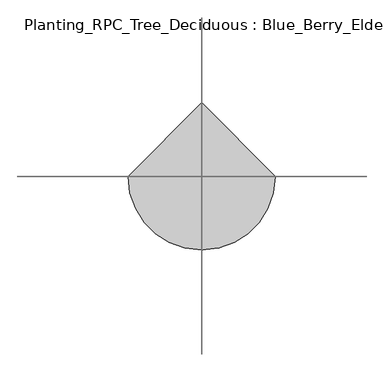
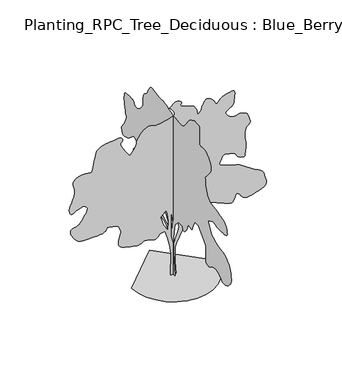
"""IFC4 building model written with IfcOpenShell, lengths in millimetres: geographic element geometry, Planting_RPC_Tree_Deciduous : Blue_Berry_Elder-4.5_Meters."""

from ifc_helpers import new_model, si_unit, origin, place, context, project, spatial, triangles, source, transform, mapped, element, save


def planting_rpc_tree_deciduous_blue_berry_elder_4_5_meters_0b743bd7(model_context):
    return source(origin(), model_context, "Body", "Tessellation", [
        triangles([(-0.0014684, 58.7037978, 0.0041346), (-0.0014684, -62.498052, 0.0041346), (-0.0014684, -15.3641626, 565.6129683), (-0.0014684, -1.8971866, 909.0182064), (-0.0014684, -22.0974929, 1104.2884094), (-0.0014684, -75.9650625, 1326.4911255), (-0.0014684, -224.1009287, 1474.6287403), (-0.0014684, -378.970291, 1474.6287403), (-0.0014684, -412.6378218, 1380.3586224), (-0.0014684, -479.9703761, 1387.0936764), (-0.0014684, -554.0404552, 1474.6287403), (-0.0014684, -601.1729708, 1568.8962421), (-0.0014684, -628.1080273, 1663.1638893), (-0.0014684, -702.1755993, 1636.2313763), (-0.0014684, -782.9756092, 1629.4963223), (-0.0014684, -857.0431812, 1797.8340122), (-0.0014684, -910.9107508, 1898.8340973), (-0.0014684, -1059.0483656, 1892.1015141), (-0.0014684, -1173.5159426, 1797.8340122), (-0.0014684, -1382.2535648, 1575.6288254), (-0.0014684, -1388.9861481, 1353.4261093), (-0.0014684, -1386.9236286, 1327.021035), (-0.0014684, -1382.3910564, 1295.553479), (-0.0014684, -1377.8561588, 1261.3760593), (-0.0014684, -1375.7936394, 1226.8434288), (-0.0014684, -1378.6786377, 1194.3159811), (-0.0014684, -1388.9861481, 1166.1459709), (-0.0014684, -1409.1860779, 1144.6884144), (-0.0014684, -1434.4711624, 1129.1809307), (-0.0014684, -1458.931152, 1117.9109064), (-0.0014684, -1483.3911415, 1111.8258854), (-0.0014684, -1508.676226, 1111.8659266), (-0.0014684, -1535.6112099, 1118.9734142), (-0.0014684, -1565.0162464, 1134.0884073), (-0.0014684, -1597.723843, 1158.1559063), (-0.0014684, -1638.2812511, 1183.6959898), (-0.0014684, -1688.0263252, 1202.5210035), (-0.0014684, -1742.9539318, 1214.5159836), (-0.0014684, -1799.0589375, 1219.5610245), (-0.0014684, -1852.3364994, 1217.541017), (-0.0014684, -1898.7841003, 1208.3335121), (-0.0014684, -1934.3939907, 1191.8234734), (-0.0014684, -1963.8416119, 1167.0484594), (-0.0014684, -1995.1716763, 1136.2684341), (-0.0014684, -2029.446619, 1104.1908863), (-0.0014684, -2067.729166, 1075.5283916), (-0.0014684, -2111.0741947, 1054.9958513), (-0.0014684, -2160.5442856, 1047.2983561), (-0.0014684, -2217.1992577, 1057.1533504), (-0.0014684, -2275.1493542, 1083.4008762), (-0.0014684, -2327.0944393, 1119.5408941), (-0.0014684, -2371.9694618, 1162.2784744), (-0.0014684, -2408.7193989, 1208.3134552), (-0.0014684, -2436.2819607, 1254.3485813), (-0.0014684, -2453.5944214, 1297.0836182), (-0.0014684, -2459.6019035, 1333.2260342), (-0.0014684, -2455.754464, 1372.7236233), (-0.0014684, -2445.3120781, 1424.1161259), (-0.0014684, -2429.919413, 1481.9887562), (-0.0014684, -2411.2318909, 1540.9212055), (-0.0014684, -2390.8944695, 1595.4962173), (-0.0014684, -2370.5569027, 1640.2937737), (-0.0014684, -2351.8669098, 1669.8963272), (-0.0014684, -2330.1568977, 1694.4363991), (-0.0014684, -2300.199424, 1725.2163517), (-0.0014684, -2262.8217636, 1758.5913494), (-0.0014684, -2218.8493023, 1790.903912), (-0.0014684, -2169.1042282, 1818.5039715), (-0.0014684, -2114.4116364, 1837.74146), (-0.0014684, -2055.5966217, 1844.9664551), (-0.0014684, -1994.4066067, 1849.8740044), (-0.0014684, -1932.1566273, 1863.6164795), (-0.0014684, -1869.0239983, 1884.7189705), (-0.0014684, -1805.1839996, 1911.7115089), (-0.0014684, -1740.8139462, 1943.1215103), (-0.0014684, -1676.0888271, 1977.4765354), (-0.0014684, -1611.1888641, 2013.3016743), (-0.0014684, -1469.786158, 2275.9068661), (-0.0014684, -1685.2562908, 2376.9094219), (-0.0014684, -1714.2713802, 2368.3093655), (-0.0014684, -1744.228854, 2360.0643745), (-0.0014684, -1776.0713871, 2352.5268986), (-0.0014684, -1810.7388931, 2346.049387), (-0.0014684, -1849.1765179, 2340.9844345), (-0.0014684, -1892.3265003, 2337.686816), (-0.0014684, -1941.1290447, 2336.5069462), (-0.0014684, -1996.881601, 2336.291843), (-0.0014684, -2057.3441895, 2336.4293346), (-0.0014684, -2118.1616982, 2338.0968201), (-0.0014684, -2174.9742188, 2342.4769306), (-0.0014684, -2223.421843, 2350.7393623), (-0.0014684, -2259.1517841, 2364.0693626), (-0.0014684, -2277.7993378, 2383.6418598), (-0.0014684, -2281.3744102, 2414.4819832), (-0.0014684, -2275.8767807, 2457.2194908), (-0.0014684, -2262.9592552, 2506.4269524), (-0.0014684, -2244.2692623, 2556.7020813), (-0.0014684, -2221.4593174, 2602.6271851), (-0.0014684, -2196.1742329, 2638.7770134), (-0.0014684, -2170.0641987, 2659.7021896), (-0.0014684, -2143.7192951, 2670.2021301), (-0.0014684, -2115.1367374, 2679.2771576), (-0.0014684, -2082.0791622, 2687.9772079), (-0.0014684, -2042.3065899, 2697.4022141), (-0.0014684, -1993.581657, 2708.6021118), (-0.0014684, -1933.6665642, 2722.6021294), (-0.0014684, -1860.326564, 2740.5021996), (-0.0014684, -1781.7239491, 2758.3022758), (-0.0014684, -1708.0688519, 2773.1522415), (-0.0014684, -1640.1838966, 2787.8522163), (-0.0014684, -1578.8962132, 2805.302314), (-0.0014684, -1525.0287163, 2828.2773651), (-0.0014684, -1479.4062103, 2859.6021973), (-0.0014684, -1442.8536449, 2902.1272179), (-0.0014684, -1414.8411106, 2953.5272781), (-0.0014684, -1393.5411026, 3009.1773697), (-0.0014684, -1377.8361019, 3068.3775352), (-0.0014684, -1366.6061188, 3130.3775299), (-0.0014684, -1358.7336342, 3194.527684), (-0.0014684, -1353.1011292, 3260.0777527), (-0.0014684, -1348.5861431, 3326.3277786), (-0.0014684, -1398.7811897, 3378.2528069), (-0.0014684, -1447.1536732, 3430.0528427), (-0.0014684, -1491.8711472, 3481.6278923), (-0.0014684, -1531.1136646, 3532.8529633), (-0.0014684, -1563.0537209, 3583.577774), (-0.0014684, -1585.8662819, 3633.7529091), (-0.0014684, -1597.723843, 3683.2030884), (-0.0014684, -1593.7188549, 3737.8779488), (-0.0014684, -1572.2812099, 3799.8529449), (-0.0014684, -1536.5912373, 3863.2281464), (-0.0014684, -1489.8311554, 3922.153038), (-0.0014684, -1435.1786774, 3970.7032722), (-0.0014684, -1375.8135509, 4002.9783371), (-0.0014684, -1314.918576, 4013.128299), (-0.0014684, -1258.4585049, 4010.1031929), (-0.0014684, -1210.3634754, 4007.7533363), (-0.0014684, -1170.7484516, 4007.6533424), (-0.0014684, -1139.7309408, 4011.3281181), (-0.0014684, -1117.4309212, 4020.3031517), (-0.0014684, -1103.9633566, 4036.1033501), (-0.0014684, -1099.4483706, 4060.2783279), (-0.0014684, -1101.1558971, 4105.3531929), (-0.0014684, -1104.8659178, 4175.1532928), (-0.0014684, -1108.4584311, 4258.1534592), (-0.0014684, -1109.8133629, 4342.8035248), (-0.0014684, -1106.8083864, 4417.5536133), (-0.0014684, -1097.3283691, 4470.8785561), (-0.0014684, -1079.2483681, 4491.2037689), (-0.0014684, -1052.7858845, 4492.578685), (-0.0014684, -1020.9033102, 4495.6035004), (-0.0014684, -985.6082989, 4498.6286064), (-0.0014684, -948.8982576, 4500.0035225), (-0.0014684, -912.7757532, 4498.07864), (-0.0014684, -879.2456778, 4491.2037689), (-0.0014684, -850.3106707, 4477.7537178), (-0.0014684, -822.8281912, 4461.7535316), (-0.0014684, -792.8706448, 4447.2035477), (-0.0014684, -761.2631264, 4432.1535942), (-0.0014684, -728.8330564, 4414.7534935), (-0.0014684, -696.4030592, 4393.1286507), (-0.0014684, -664.7980116, 4365.3786003), (-0.0014684, -634.8405378, 4329.6034584), (-0.0014684, -604.8054889, 4286.4284775), (-0.0014684, -572.6504748, 4239.8534134), (-0.0014684, -538.7279451, 4193.0283646), (-0.0014684, -503.3904219, 4149.1534264), (-0.0014684, -466.9953687, 4111.403405), (-0.0014684, -429.8928369, 4082.9533974), (-0.0014684, -392.4378193, 4067.0032082), (-0.0014684, -354.0977903, 4061.0282822), (-0.0014684, -314.1102602, 4059.6533661), (-0.0014684, -272.4727218, 4061.703241), (-0.0014684, -229.1851932, 4065.9782707), (-0.0014684, -184.2498909, 4071.3282349), (-0.0014684, -137.6653616, 4076.5532066), (-0.0014684, -89.4320684, 4080.4782578), (-0.0014684, -32.5020268, 4087.803392), (-0.0014684, 35.3820291, 4102.1033913), (-0.0014684, 107.0353362, 4120.403437), (-0.0014684, 175.2726409, 4139.7534187), (-0.0014684, 232.909439, 4157.2282242), (-0.0014684, 272.7602224, 4169.8783241), (-0.0014684, 287.6402371, 4174.7283188), (-0.0014684, 295.8277461, 4177.2784538), (-0.0014684, 318.5002539, 4183.6033585), (-0.0014684, 352.8352947, 4191.7034454), (-0.0014684, 396.002827, 4199.553257), (-0.0014684, 445.1803485, 4205.1534966), (-0.0014684, 497.5354013, 4206.5284126), (-0.0014684, 550.2454471, 4201.678418), (-0.0014684, 608.3329988, 4200.728476), (-0.0014684, 675.2555128, 4211.4534027), (-0.0014684, 745.8280947, 4228.1785446), (-0.0014684, 814.8706827, 4245.2533745), (-0.0014684, 877.2007444, 4257.0285278), (-0.0014684, 927.6307331, 4257.8534775), (-0.0014684, 960.9857466, 4242.0785683), (-0.0014684, 983.9932812, 4214.9534798), (-0.0014684, 1006.5283155, 4185.8035149), (-0.0014684, 1028.1233637, 4155.1533508), (-0.0014684, 1048.3033819, 4123.4282524), (-0.0014684, 1066.5983408, 4091.1031906), (-0.0014684, 1082.5408997, 4058.6781349), (-0.0014684, 1095.6533987, 4026.6033485), (-0.0014684, 1111.3184309, 3999.2282753), (-0.0014684, 1133.5808802, 3978.353096), (-0.0014684, 1159.9634268, 3960.5283119), (-0.0014684, 1187.9984888, 3942.3532585), (-0.0014684, 1215.2059851, 3920.4031448), (-0.0014684, 1239.1159355, 3891.2531799), (-0.0014684, 1257.255962, 3851.5279884), (-0.0014684, 1268.2685165, 3817.1530518), (-0.0014684, 1273.6285091, 3800.8031776), (-0.0014684, 1275.1010937, 3794.1030052), (-0.0014684, 1274.4534588, 3788.7030441), (-0.0014684, 1273.451049, 3776.252932), (-0.0014684, 1273.8635239, 3748.3528908), (-0.0014684, 1277.4560371, 3696.6528488), (-0.0014684, 1283.7985279, 3637.6029648), (-0.0014684, 1291.9060272, 3591.1778915), (-0.0014684, 1302.7210648, 3554.2528198), (-0.0014684, 1317.1884956, 3523.8279327), (-0.0014684, 1336.2511402, 3496.8278366), (-0.0014684, 1360.8486214, 3470.1527206), (-0.0014684, 1391.9260849, 3440.8027679), (-0.0014684, 1427.2211689, 3411.5778076), (-0.0014684, 1463.2262386, 3387.677813), (-0.0014684, 1498.9912067, 3369.4027657), (-0.0014684, 1533.5812466, 3357.1526413), (-0.0014684, 1566.0512123, 3351.2777092), (-0.0014684, 1595.4587196, 3352.1026588), (-0.0014684, 1620.8612389, 3360.002758), (-0.0014684, 1639.7087803, 3375.502684), (-0.0014684, 1652.8988182, 3396.6528465), (-0.0014684, 1664.6789131, 3420.0528717), (-0.0014684, 1679.2838356, 3442.2776779), (-0.0014684, 1700.9563499, 3459.9027649), (-0.0014684, 1733.936459, 3469.5277588), (-0.0014684, 1782.4638748, 3467.7278687), (-0.0014684, 1840.5514629, 3464.2277916), (-0.0014684, 1897.5815575, 3466.9779144), (-0.0014684, 1950.8390625, 3469.852739), (-0.0014684, 1997.6216721, 3466.7029312), (-0.0014684, 2035.2141449, 3451.4277008), (-0.0014684, 2060.9117043, 3417.9027122), (-0.0014684, 2072.001725, 3360.002758), (-0.0014684, 2074.396637, 3302.2527946), (-0.0014684, 2075.4967152, 3266.6526421), (-0.0014684, 2074.8291687, 3243.2026199), (-0.0014684, 2071.9241135, 3221.8774681), (-0.0014684, 2066.3091946, 3192.6275093), (-0.0014684, 2057.5140919, 3145.5024788), (-0.0014684, 2045.069212, 3070.4524086), (-0.0014684, 2028.7941879, 2993.7774376), (-0.0014684, 2011.3440903, 2941.8274109), (-0.0014684, 1996.4816254, 2904.7273499), (-0.0014684, 1987.9815628, 2872.5772774), (-0.0014684, 1989.6115505, 2835.4772163), (-0.0014684, 2005.1390911, 2783.5271896), (-0.0014684, 2038.3341579, 2706.8522186), (-0.0014684, 2081.1517479, 2626.4521843), (-0.0014684, 2121.139278, 2566.6770538), (-0.0014684, 2155.4742462, 2522.5771294), (-0.0014684, 2181.326738, 2489.1794586), (-0.0014684, 2195.8742512, 2461.5570168), (-0.0014684, 2196.286726, 2434.7619953), (-0.0014684, 2179.7367187, 2403.841935), (-0.0014684, 2160.4392048, 2371.8244125), (-0.0014684, 2149.859182, 2345.5768867), (-0.0014684, 2141.0441677, 2325.9269234), (-0.0014684, 2127.0467663, 2313.6968559), (-0.0014684, 2100.919146, 2309.7119247), (-0.0014684, 2055.7091148, 2314.7969341), (-0.0014684, 1984.4666611, 2329.7743629), (-0.0014684, 1906.7291096, 2358.6118469), (-0.0014684, 1844.06651, 2399.6994553), (-0.0014684, 1792.5939251, 2445.4995667), (-0.0014684, 1748.4239468, 2488.4719437), (-0.0014684, 1707.671347, 2521.0769302), (-0.0014684, 1666.4437763, 2535.7769051), (-0.0014684, 1620.8612389, 2525.0519783), (-0.0014684, 1576.9088345, 2499.6619583), (-0.0014684, 1542.1411892, 2475.3396057), (-0.0014684, 1515.031216, 2451.8994667), (-0.0014684, 1494.0461597, 2429.166988), (-0.0014684, 1477.653701, 2406.9644188), (-0.0014684, 1464.3237007, 2385.1144444), (-0.0014684, 1452.526165, 2363.44193), (-0.0014684, 1471.2737125, 2344.7718487), (-0.0014684, 1489.9612347, 2326.6344383), (-0.0014684, 1508.5336475, 2309.5543762), (-0.0014684, 1526.9262749, 2294.0668041), (-0.0014684, 1545.0862129, 2280.6968353), (-0.0014684, 1562.9512562, 2269.9793209), (-0.0014684, 1580.4612339, 2262.4393742), (-0.0014684, 1599.1313152, 2259.024321), (-0.0014684, 1619.331245, 2258.1993713), (-0.0014684, 1639.2963055, 2256.7868122), (-0.0014684, 1657.2588718, 2251.6042797), (-0.0014684, 1671.4513195, 2239.4718807), (-0.0014684, 1680.1087852, 2217.2092861), (-0.0014684, 1681.4637897, 2181.6392189), (-0.0014684, 1676.9863014, 2141.9842266), (-0.0014684, 1669.5664055, 2107.6292015), (-0.0014684, 1659.5537899, 2075.631736), (-0.0014684, 1647.3038109, 2043.0441902), (-0.0014684, 1633.1713886, 2006.9216858), (-0.0014684, 1617.5037403, 1964.3241405), (-0.0014684, 1600.6613091, 1912.3015892), (-0.0014684, 1583.268766, 1853.7415009), (-0.0014684, 1567.0537674, 1795.0639778), (-0.0014684, 1554.0188072, 1738.6264343), (-0.0014684, 1546.1662342, 1686.7788723), (-0.0014684, 1545.4986877, 1641.8837929), (-0.0014684, 1554.0188072, 1606.2938141), (-0.0014684, 1573.728796, 1582.3637341), (-0.0014684, 1599.1112583, 1566.4212479), (-0.0014684, 1623.4337563, 1552.9562267), (-0.0014684, 1646.8738953, 1541.5487835), (-0.0014684, 1669.606374, 1531.7937103), (-0.0014684, 1691.8087978, 1523.2737362), (-0.0014684, 1713.6589176, 1515.5787117), (-0.0014684, 1735.331432, 1508.2936913), (-0.0014684, 1758.2389, 1518.0512352), (-0.0014684, 1780.0888744, 1525.7462597), (-0.0014684, 1799.8189201, 1529.318716), (-0.0014684, 1816.3664566, 1526.7087009), (-0.0014684, 1828.676461, 1515.8536949), (-0.0014684, 1835.6840275, 1494.6911785), (-0.0014684, 1836.331517, 1461.1612484), (-0.0014684, 1830.501495, 1425.4711304), (-0.0014684, 1819.3715057, 1398.2636341), (-0.0014684, 1803.8239082, 1378.1211136), (-0.0014684, 1784.7414974, 1363.6336258), (-0.0014684, 1763.0089577, 1353.3861408), (-0.0014684, 1739.5114094, 1345.9660995), (-0.0014684, 1715.128886, 1339.9586174), (-0.0014684, 1703.5663651, 1332.6360992), (-0.0014684, 1691.8864094, 1324.6660915), (-0.0014684, 1679.9712936, 1315.4011047), (-0.0014684, 1667.701403, 1304.1910332), (-0.0014684, 1654.9613377, 1290.3910034), (-0.0014684, 1641.6313374, 1273.3510551), (-0.0014684, 1627.5962929, 1252.4235535), (-0.0014684, 1608.2588104, 1230.1234612), (-0.0014684, 1580.0887276, 1209.2360006), (-0.0014684, 1544.5563034, 1189.5259392), (-0.0014684, 1503.1336864, 1170.7584801), (-0.0014684, 1457.2962227, 1152.6984632), (-0.0014684, 1408.5135899, 1135.1084032), (-0.0014684, 1358.2586632, 1117.7559013), (-0.0014684, 1196.6559546, 1212.0234758), (-0.0014684, 1035.0533186, 1090.8208448), (-0.0014684, 1013.4382862, 1088.0133854), (-0.0014684, 992.0007866, 1085.6783535), (-0.0014684, 970.9182798, 1084.2833805), (-0.0014684, 950.3632845, 1084.3033648), (-0.0014684, 930.5182749, 1086.2084084), (-0.0014684, 911.5532261, 1090.4683954), (-0.0014684, 893.6507578, 1097.5558989), (-0.0014684, 877.0431959, 1106.938393), (-0.0014684, 861.3756929, 1117.3809242), (-0.0014684, 845.9456755, 1128.295883), (-0.0014684, 830.0457012, 1139.0934071), (-0.0014684, 812.9656391, 1149.1834162), (-0.0014684, 794.0031338, 1157.9784462), (-0.0014684, 772.4481268, 1164.8884169), (-0.0014684, 748.1855816, 1170.2684664), (-0.0014684, 721.8005642, 1174.9409283), (-0.0014684, 693.6505383, 1179.0234552), (-0.0014684, 664.0855551, 1182.6359528), (-0.0014684, 633.4605349, 1185.8934574), (-0.0014684, 602.1304705, 1188.9184908), (-0.0014684, 570.4454495, 1191.8234734), (-0.0014684, 361.7077909, 1131.2209225), (-0.0014684, 186.6391528, 1003.2857809), (-0.0014684, 92.3710787, 848.418199), (-0.0014684, 45.2367873, 552.1454401), (-0.0013758, 65.4370532, 1097.5558989), (-0.0013758, 166.4388778, 1313.0261044), (-0.0013758, 4.8361539, 1380.3586224), (-0.0013882, 307.8402577, 1171.6234709), (-0.0013882, 469.4428937, 1279.3585373), (-0.0013882, 597.3779989, 1286.0909752), (-0.0013882, 705.1130653, 1346.6910553), (-0.0013882, 699.3031002, 1349.8135391), (-0.0013882, 693.2555769, 1354.3485821), (-0.0013882, 686.7405676, 1361.7110687), (-0.0013882, 679.5155725, 1373.3110874), (-0.0013882, 671.3480478, 1390.5686096), (-0.0013882, 662.0055222, 1414.8911076), (-0.0013882, 651.2454958, 1447.6936111), (-0.0013882, 642.6479828, 1480.1036968), (-0.0013882, 639.3505096, 1503.3287327), (-0.0013882, 640.4680286, 1518.8962418), (-0.0013882, 645.1205063, 1528.3386887), (-0.0013882, 652.425511, 1533.1862125), (-0.0013882, 661.4930534, 1534.9737488), (-0.0013882, 671.4480417, 1535.2286751), (-0.0013882, 678.1805523, 1616.0288303), (-0.0013882, 597.3779989, 1669.8963272), (-0.0013882, 422.3103418, 1521.7611832), (-0.0013882, 301.1077472, 1380.3586224), (-0.0013882, 220.3061749, 1265.8910454), (-0.0013882, 139.504866, 1084.0884069), (66.6360534, 0.0002629, 0.0), (-68.0330566, 0.0002629, 0.0), (-61.2998012, 0.0002272, 552.142933), (-94.9670776, 0.0002139, 794.5456152), (-142.1008648, 0.0002005, 996.5483288), (-202.7016716, 0.0001916, 1178.3509672), (-323.9027584, 0.0001916, 1164.8859461), (-344.1627863, 0.0001916, 1136.3209019), (-364.7752999, 0.000196, 1109.5258804), (-386.0953285, 0.000196, 1086.2633469), (-408.4753215, 0.000196, 1068.3008532), (-432.2678372, 0.0002005, 1057.4058786), (-457.8253615, 0.0002005, 1055.3433592), (-485.5053944, 0.000196, 1063.8833902), (-514.9529065, 0.000196, 1076.7408903), (-545.4604557, 0.000196, 1086.7733448), (-576.8504728, 0.000196, 1094.448385), (-608.9454978, 0.000196, 1100.2409094), (-641.5730484, 0.000196, 1104.6184038), (-674.5530121, 0.000196, 1108.0533686), (-707.7105812, 0.000196, 1111.0183765), (-735.2131176, 0.000196, 1095.3133759), (-763.2456362, 0.000196, 1080.6083868), (-792.3406626, 0.000196, 1067.9083626), (-823.0231647, 0.000196, 1058.210844), (-855.8256683, 0.0002005, 1052.5183863), (-891.280699, 0.0002005, 1051.8308556), (-929.9132246, 0.0002005, 1057.1508797), (-979.8558157, 0.000196, 1066.7883728), (-1044.1658438, 0.000196, 1079.0183676), (-1115.7808765, 0.000196, 1094.7833937), (-1187.630924, 0.000196, 1115.0233646), (-1252.6485397, 0.0001916, 1140.6809555), (-1303.7660591, 0.0001916, 1172.6984779), (-1333.9185791, 0.0001871, 1212.0184616), (-1343.6560661, 0.0001871, 1258.8785374), (-1340.9085594, 0.0001827, 1310.6835148), (-1329.6785763, 0.0001782, 1364.141153), (-1313.9735756, 0.0001782, 1415.9461304), (-1297.7985455, 0.0001738, 1462.8062061), (-1285.1560032, 0.0001738, 1501.4186749), (-1280.0510822, 0.0001693, 1528.4912956), (-1282.3885849, 0.0001693, 1551.6362492), (-1288.8460396, 0.0001693, 1579.2562202), (-1298.6035835, 0.0001648, 1609.2337509), (-1310.8335056, 0.0001648, 1639.4462963), (-1324.7136177, 0.0001604, 1667.7737823), (-1339.4160633, 0.0001604, 1692.0964256), (-1354.121125, 0.0001604, 1710.2938614), (-1373.4561367, 0.0001604, 1723.3488785), (-1401.6286903, 0.0001559, 1733.9289013), (-1437.1586437, 0.0001559, 1742.4488754), (-1478.5812607, 0.0001559, 1749.3189503), (-1524.4187244, 0.0001559, 1754.9539261), (-1573.2012119, 0.0001559, 1759.7639523), (-1623.456284, 0.0001559, 1764.1613583), (-1631.2713593, 0.0001559, 1738.3664211), (-1642.6763317, 0.0001604, 1713.6314484), (-1661.2663307, 0.0001604, 1691.0164043), (-1690.6363403, 0.0001604, 1671.5813988), (-1734.3739323, 0.0001604, 1656.386396), (-1796.0739452, 0.0001648, 1646.4938313), (-1879.3290379, 0.0001648, 1642.9588726), (-1971.5741341, 0.0001648, 1640.6613384), (-2057.4616241, 0.0001648, 1636.1262955), (-2136.396777, 0.0001648, 1632.8888477), (-2207.7943085, 0.0001648, 1634.478867), (-2271.0668999, 0.0001648, 1644.4313118), (-2325.619384, 0.0001604, 1666.2812862), (-2370.8693836, 0.0001604, 1703.5614235), (-2411.8019142, 0.0001559, 1752.5588688), (-2450.9643494, 0.0001559, 1805.3264328), (-2484.1219185, 0.0001515, 1859.0389973), (-2507.0269157, 0.000147, 1910.8640316), (-2515.4519829, 0.0001426, 1957.9790337), (-2505.1520302, 0.0001426, 1997.554089), (-2471.8720848, 0.0001426, 2026.7640793), (-2428.4670307, 0.0001381, 2045.1192089), (-2390.1269291, 0.0001381, 2056.5266521), (-2356.1468811, 0.0001381, 2064.7517315), (-2325.816901, 0.0001381, 2073.5667458), (-2298.4317993, 0.0001381, 2086.7391975), (-2273.2843517, 0.0001337, 2108.0367348), (-2249.6667526, 0.0001337, 2141.2342724), (-2221.7142437, 0.0001292, 2184.9518074), (-2187.6342018, 0.0001292, 2233.7342949), (-2152.8467903, 0.0001247, 2285.2267914), (-2122.7717365, 0.0001203, 2337.0718826), (-2102.826733, 0.0001203, 2386.9169506), (-2098.4291817, 0.0001158, 2432.401965), (-2114.9992458, 0.0001158, 2471.1721275), (-2145.426749, 0.0001114, 2498.537027), (-2178.6816959, 0.0001114, 2512.8271431), (-2214.2917316, 0.0001114, 2516.2269356), (-2251.7868267, 0.0001114, 2510.9019699), (-2290.6968063, 0.0001114, 2499.0494957), (-2330.5468449, 0.0001114, 2482.831881), (-2370.8693836, 0.0001158, 2464.439399), (-2399.569376, 0.0001158, 2448.8118645), (-2427.3294548, 0.0001158, 2434.6595306), (-2453.2020035, 0.0001158, 2423.4494591), (-2476.2471085, 0.0001158, 2416.6569958), (-2495.5270363, 0.0001158, 2415.7544346), (-2510.1020187, 0.0001158, 2422.2118893), (-2519.0020569, 0.0001158, 2437.5044151), (-2525.7269371, 0.0001158, 2456.4494797), (-2533.1520653, 0.0001158, 2474.4518692), (-2539.5019684, 0.0001114, 2493.8669632), (-2543.0270439, 0.0001114, 2517.0521759), (-2541.977108, 0.0001114, 2546.3521317), (-2534.5519798, 0.0001069, 2584.15215), (-2519.0020569, 0.0001025, 2632.7770889), (-2498.1969315, 0.0001025, 2684.6521202), (-2477.0345604, 9.8e-05, 2732.0771324), (-2456.8145737, 9.8e-05, 2777.1272896), (-2438.8319504, 9.36e-05, 2821.9271713), (-2424.3844311, 8.91e-05, 2868.6522263), (-2414.7643787, 8.91e-05, 2919.3523293), (-2411.2693886, 8.47e-05, 2976.1773491), (-2415.2169674, 8.02e-05, 3030.6775108), (-2424.696912, 8.02e-05, 3074.9274261), (-2436.1819668, 7.57e-05, 3111.8774963), (-2446.1344116, 7.57e-05, 3144.4525429), (-2451.0245201, 7.13e-05, 3175.6276749), (-2447.311956, 7.13e-05, 3208.3277138), (-2431.4719345, 6.68e-05, 3245.527478), (-2401.6519524, 6.68e-05, 3281.1526291), (-2361.1144558, 6.24e-05, 3307.9527374), (-2313.9793968, 6.24e-05, 3326.977739), (-2264.3718143, 6.24e-05, 3339.2775696), (-2216.4142765, 6.24e-05, 3345.9277451), (-2174.2267353, 6.24e-05, 3348.0026184), (-2141.9342297, 6.24e-05, 3346.5277084), (-2114.2341763, 6.24e-05, 3341.002755), (-2084.4141941, 6.24e-05, 3332.902668), (-2054.4766319, 6.24e-05, 3326.2027863), (-2026.4241291, 6.24e-05, 3324.9275734), (-2002.2565636, 6.24e-05, 3333.0776573), (-1983.9816616, 6.24e-05, 3354.6527939), (-1973.5965397, 5.79e-05, 3393.652739), (-1964.8216393, 5.35e-05, 3450.0277863), (-1951.2165104, 5.35e-05, 3517.3777451), (-1934.5515392, 4.9e-05, 3590.1279556), (-1916.5891182, 4.46e-05, 3662.7528831), (-1899.0965813, 4.01e-05, 3729.7281555), (-1883.8440239, 3.56e-05, 3785.5279472), (-1872.5939838, 3.12e-05, 3824.6031784), (-1852.5114887, 3.12e-05, 3852.8781967), (-1813.3489082, 3.12e-05, 3879.4030312), (-1760.7564789, 2.67e-05, 3903.2280304), (-1700.3914135, 2.67e-05, 3923.3782539), (-1637.906274, 2.67e-05, 3938.9531754), (-1578.9537678, 2.67e-05, 3948.9781448), (-1529.1887821, 2.67e-05, 3952.5282188), (-1482.7811497, 2.67e-05, 3955.978299), (-1432.4861092, 2.67e-05, 3963.6781197), (-1381.8386192, 2.67e-05, 3971.6032173), (-1334.3710224, 2.23e-05, 3975.7782532), (-1293.6160973, 2.67e-05, 3972.1531837), (-1263.1109825, 2.67e-05, 3956.7782501), (-1246.3835152, 2.67e-05, 3925.6031181), (-1245.9735111, 3.12e-05, 3891.2531799), (-1257.1035004, 3.12e-05, 3865.2780212), (-1272.3560577, 3.12e-05, 3842.0279869), (-1284.3134674, 3.56e-05, 3815.8281326), (-1285.5485664, 3.56e-05, 3781.0029327), (-1268.6459644, 4.01e-05, 3731.9530197), (-1226.1860561, 4.46e-05, 3663.0028679), (-1175.7534513, 4.9e-05, 3589.303006), (-1137.6884056, 4.9e-05, 3530.2028343), (-1108.6933731, 5.35e-05, 3486.3028976), (-1085.4708807, 5.35e-05, 3458.2028687), (-1064.7208391, 5.79e-05, 3446.4527138), (-1043.1458479, 5.35e-05, 3451.6776855), (-1017.4482885, 5.35e-05, 3474.4527489), (-990.2407923, 5.35e-05, 3507.3527756), (-966.3282984, 4.9e-05, 3542.2529709), (-945.7157484, 4.9e-05, 3578.7027809), (-928.403215, 4.46e-05, 3616.2028175), (-914.3857567, 4.46e-05, 3654.2778191), (-903.6682423, 4.01e-05, 3692.4781036), (-896.2457302, 4.01e-05, 3730.3281189), (-882.6607309, 3.56e-05, 3773.9530724), (-855.1781788, 3.12e-05, 3826.1530838), (-816.3881773, 3.12e-05, 3881.5531906), (-768.880612, 2.67e-05, 3934.7281425), (-715.2480572, 2.23e-05, 3980.2282722), (-658.0830145, 2.23e-05, 4012.6533279), (-599.9754785, 2.23e-05, 4026.6033485), (-552.8204352, 2.23e-05, 4024.7781693), (-521.215424, 2.23e-05, 4016.1031174), (-496.7928958, 2.23e-05, 4004.503244), (-471.1953667, 2.23e-05, 3993.8533127), (-436.0553604, 2.23e-05, 3988.0280869), (-383.0128132, 2.23e-05, 3990.9032021), (-303.7027378, 2.23e-05, 4006.4031281), (-214.7551692, 2.23e-05, 4026.5783501), (-138.763614, 2.23e-05, 4042.5282486), (-76.3173075, 1.78e-05, 4056.5782631), (-28.0055217, 1.78e-05, 4071.1032486), (5.5830293, 1.78e-05, 4088.4533524), (23.8594698, 1.78e-05, 4110.9784309), (26.2347722, 1.34e-05, 4141.0533394), (18.3040142, 1.34e-05, 4173.7283798), (6.4862053, 8.9e-06, 4202.8533463), (-8.5707069, 8.9e-06, 4229.0534912), (-26.219021, 8.9e-06, 4252.8784904), (-45.810535, 4.5e-06, 4274.9535965), (-66.6978047, 4.5e-06, 4295.8284851), (-88.2330682, 4.5e-06, 4316.1284088), (-60.8870493, 4.5e-06, 4341.9035797), (-33.9532782, 0.0, 4366.5035316), (-7.8441564, 0.0, 4388.753627), (17.0283143, 0.0, 4407.4536484), (40.2517809, 0.0, 4421.4536659), (61.4140475, -4.5e-06, 4429.5534622), (80.1028141, -4.5e-06, 4430.6036888), (99.5373291, -4.5e-06, 4426.853627), (121.7990971, 0.0, 4421.2286797), (144.7671174, 0.0, 4413.4535728), (166.3221335, 0.0, 4403.3536079), (184.343399, 0.0, 4390.653511), (196.7109036, 0.0, 4375.1285866), (201.3046639, 0.0, 4356.5285591), (197.1231604, 4.5e-06, 4339.6534264), (187.641399, 4.5e-06, 4327.8285667), (177.4531401, 4.5e-06, 4318.7285408), (171.1516352, 4.5e-06, 4309.9784935), (173.3306447, 4.5e-06, 4299.2035698), (188.5839106, 4.5e-06, 4284.1033287), (221.5051751, 8.9e-06, 4262.2784981), (265.7927153, 8.9e-06, 4240.0534012), (311.140238, 8.9e-06, 4223.8285194), (356.135275, 8.9e-06, 4211.3784073), (399.3628326, 8.9e-06, 4200.4784912), (439.4103518, 1.34e-05, 4188.8533287), (474.8628754, 1.34e-05, 4174.2783463), (504.3104239, 1.34e-05, 4154.528389), (527.7304333, 1.34e-05, 4129.0781982), (546.555447, 1.78e-05, 4099.4032654), (561.5529691, 1.78e-05, 4066.203257), (573.4879601, 2.23e-05, 4030.1531319), (583.1279603, 2.23e-05, 3991.9781364), (591.2354596, 2.67e-05, 3952.4032265), (598.5779984, 2.67e-05, 3912.1280685), (692.8455729, 2.23e-05, 3999.6532494), (692.2180676, 2.23e-05, 4003.2033234), (691.118062, 2.23e-05, 4013.1033005), (690.7255714, 2.23e-05, 4028.2782463), (692.2180676, 2.23e-05, 4047.7282219), (696.7730947, 1.78e-05, 4070.3282959), (705.5680521, 1.78e-05, 4095.0782387), (719.7805567, 1.78e-05, 4120.8534096), (736.0730942, 1.34e-05, 4147.7032242), (751.1906307, 1.34e-05, 4174.7783157), (766.4231312, 8.9e-06, 4199.8285309), (783.0706615, 8.9e-06, 4220.678421), (802.4256575, 8.9e-06, 4235.0284172), (825.7856415, 8.9e-06, 4240.6533646), (854.4482088, 8.9e-06, 4235.3283989), (884.2282225, 8.9e-06, 4222.4283142), (910.4757483, 8.9e-06, 4207.0283821), (933.7782503, 1.34e-05, 4189.5782845), (954.7232655, 1.34e-05, 4170.4782875), (973.9032721, 1.34e-05, 4150.1283669), (991.9033361, 1.34e-05, 4128.9782043), (1009.3183342, 1.78e-05, 4107.4033585), (1013.7732948, 1.78e-05, 4086.0282097), (1018.9957958, 1.78e-05, 4066.2282555), (1025.7483633, 1.78e-05, 4049.6283966), (1034.7983196, 2.23e-05, 4037.7782478), (1046.9108797, 2.23e-05, 4032.3032913), (1062.8508224, 2.23e-05, 4034.7781403), (1083.3859062, 2.23e-05, 4046.8032784), (1105.9034271, 1.78e-05, 4067.7281639), (1128.3008972, 1.78e-05, 4093.828315), (1152.1133972, 1.78e-05, 4122.0533363), (1178.8709209, 1.34e-05, 4149.3534142), (1210.1034622, 1.34e-05, 4172.628447), (1247.3434856, 1.34e-05, 4188.8533287), (1292.120985, 1.34e-05, 4194.9282486), (1340.4335884, 8.9e-06, 4200.0785156), (1385.9186028, 8.9e-06, 4211.3534088), (1426.5736794, 8.9e-06, 4222.5033096), (1460.3986496, 8.9e-06, 4227.2783089), (1485.388694, 8.9e-06, 4219.4784943), (1499.543644, 1.34e-05, 4192.8033783), (1500.85868, 1.34e-05, 4141.0533394), (1496.0287422, 1.78e-05, 4077.6284317), (1491.9061741, 2.23e-05, 4020.1781593), (1486.7236416, 2.67e-05, 3968.9780869), (1478.7161362, 2.67e-05, 3924.2532005), (1466.111237, 3.12e-05, 3886.2531944), (1447.1487316, 3.12e-05, 3855.2030548), (1420.05867, 3.12e-05, 3831.3280586), (1386.1536175, 3.56e-05, 3811.7280922), (1350.8386219, 3.56e-05, 3792.5031029), (1318.4660339, 3.56e-05, 3772.3281715), (1293.3985233, 3.56e-05, 3749.9030869), (1279.9910568, 4.01e-05, 3723.9529266), (1282.6010719, 4.01e-05, 3693.1530624), (1305.5886223, 4.46e-05, 3656.2529892), (1339.7660419, 4.46e-05, 3620.9528183), (1372.8836426, 4.9e-05, 3594.8529579), (1404.7061188, 4.9e-05, 3576.4029213), (1434.9961304, 4.9e-05, 3564.0778015), (1463.5211334, 4.9e-05, 3556.3279839), (1490.0411716, 4.9e-05, 3551.6529785), (1514.3261719, 4.9e-05, 3548.5278786), (1534.9188103, 4.9e-05, 3550.0027885), (1552.0962502, 4.9e-05, 3557.8278923), (1568.2112549, 4.9e-05, 3568.4778236), (1585.6263256, 4.9e-05, 3578.4527962), (1606.6888481, 4.9e-05, 3584.1530296), (1633.7613235, 4.9e-05, 3582.1028641), (1669.1938992, 4.9e-05, 3568.7278084), (1706.7689312, 4.9e-05, 3552.8279068), (1738.9239452, 4.9e-05, 3542.9279297), (1766.0138615, 4.9e-05, 3535.1528229), (1788.3938908, 4.9e-05, 3525.6028244), (1806.4140118, 5.35e-05, 3510.4278786), (1820.4314701, 5.35e-05, 3485.6779358), (1830.7965351, 5.79e-05, 3447.5276482), (1843.1639488, 5.79e-05, 3405.1526184), (1859.6539307, 6.24e-05, 3369.1527809), (1875.3189629, 6.24e-05, 3337.6276703), (1885.2139984, 6.24e-05, 3308.7026917), (1884.3890488, 6.68e-05, 3280.4526718), (1867.8990669, 6.68e-05, 3251.0527222), (1830.7965351, 7.13e-05, 3218.5776695), (1790.6914249, 7.13e-05, 3174.2274696), (1766.368927, 7.57e-05, 3114.4526299), (1754.6488575, 8.02e-05, 3045.2524933), (1752.3514687, 8.47e-05, 2972.6522736), (1756.2964314, 8.91e-05, 2902.627478), (1763.3064686, 9.36e-05, 2841.2021576), (1770.196455, 9.36e-05, 2794.3773994), (1774.2014431, 9.8e-05, 2756.2771088), (1775.0263927, 9.8e-05, 2717.1021744), (1773.198888, 0.0001025, 2677.0522934), (1769.2539253, 0.0001025, 2636.3021645), (1763.7189434, 0.0001069, 2595.0270676), (1757.121381, 0.0001069, 2553.3769936), (1749.9963799, 0.0001114, 2511.5769287), (1751.0764011, 0.0001114, 2490.1945129), (1749.9764683, 0.0001158, 2470.407058), (1744.5189526, 0.0001158, 2453.7993507), (1732.5238998, 0.0001158, 2441.9619919), (1711.8138268, 0.0001158, 2436.4844193), (1680.2063084, 0.0001158, 2438.9569427), (1635.5263321, 0.0001158, 2450.971907), (1592.8687614, 0.0001158, 2472.329615), (1564.6988239, 0.0001114, 2499.8145653), (1544.891312, 0.0001114, 2530.4769379), (1527.3211636, 0.0001069, 2561.3770866), (1505.8637524, 0.0001069, 2589.5771095), (1474.3961964, 0.0001069, 2612.1021881), (1426.7911079, 0.0001069, 2626.0522087), (1373.8061153, 0.0001025, 2635.8521919), (1329.4210339, 0.0001025, 2646.0271523), (1292.338559, 0.0001025, 2653.6022713), (1261.2609501, 0.0001025, 2655.6521461), (1234.8984604, 0.0001025, 2649.2022491), (1211.9484804, 0.0001025, 2631.3521759), (1191.1209726, 0.0001069, 2599.1021095), (1170.9584679, 0.0001069, 2559.6521919), (1152.6834206, 0.0001114, 2522.5521309), (1139.0008982, 0.0001114, 2488.5071159), (1132.6209097, 0.0001158, 2458.2345451), (1136.2509207, 0.0001158, 2432.4394627), (1152.6034109, 0.0001158, 2411.8269127), (1184.3859913, 0.0001203, 2397.1044102), (1219.3110397, 0.0001203, 2386.6219105), (1246.1060612, 0.0001203, 2377.5519699), (1269.016, 0.0001203, 2368.8369495), (1292.2785336, 0.0001203, 2359.4119434), (1320.1361355, 0.0001203, 2348.2243996), (1356.8260471, 0.0001203, 2334.2069412), (1406.5911781, 0.0001247, 2316.3044003), (1459.7312485, 0.0001247, 2299.7343361), (1505.2162628, 0.0001247, 2288.4668552), (1545.2837299, 0.0001247, 2279.5543179), (1582.1713039, 0.0001247, 2270.0518456), (1618.1138775, 0.0001247, 2257.0168854), (1655.3539009, 0.0001292, 2237.5042683), (1696.128883, 0.0001292, 2208.5692612), (1938.5315289, 0.0001381, 2040.2317165), (1981.0741356, 0.0001426, 2013.7116783), (2030.6815727, 0.0001426, 1989.6615475), (2082.8791134, 0.0001426, 1964.7890831), (2133.1942108, 0.000147, 1935.7940506), (2177.1467606, 0.000147, 1899.3789768), (2210.2642159, 0.0001515, 1852.246534), (2228.0692337, 0.0001559, 1791.0940166), (2241.2617424, 0.0001604, 1726.50886), (2258.5768192, 0.0001604, 1670.1688396), (2272.5942776, 0.0001648, 1620.4237656), (2275.8918961, 0.0001693, 1575.6237385), (2261.0493427, 0.0001693, 1534.1238007), (2220.6493378, 0.0001738, 1494.2737621), (2147.2692238, 0.0001738, 1454.4237236), (2059.4391197, 0.0001782, 1418.5387047), (1980.5616669, 0.0001782, 1391.6035755), (1910.5189945, 0.0001782, 1373.5036629), (1849.1914879, 0.0001782, 1364.121096), (1796.4614216, 0.0001782, 1363.3361149), (1752.2139771, 0.0001782, 1371.0311394), (1716.3289581, 0.0001782, 1387.0885895), (1685.0163345, 0.0001782, 1414.9836891), (1654.6488567, 0.0001738, 1452.773679), (1625.3388725, 0.0001738, 1492.2137135), (1597.2087582, 0.0001693, 1525.0561855), (1570.3712975, 0.0001693, 1543.0562496), (1544.9487213, 0.0001693, 1537.973711), (1521.0587551, 0.0001738, 1501.5561665), (1500.85868, 0.0001738, 1451.6536892), (1484.7811729, 0.0001782, 1411.5286674), (1470.3512398, 0.0001782, 1381.0610504), (1455.0986824, 0.0001782, 1360.1361649), (1436.5486519, 0.0001827, 1348.6310532), (1412.2236832, 0.0001827, 1346.4336582), (1379.656049, 0.0001827, 1353.4210224), (1340.768597, 0.0001782, 1366.1410309), (1299.4060055, 0.0001782, 1380.9835842), (1255.9810398, 0.0001782, 1397.5911461), (1210.9085003, 0.0001782, 1415.6111217), (1164.5984636, 0.0001738, 1434.6936779), (1117.4658754, 0.0001738, 1454.4811329), (1069.9183416, 0.0001738, 1474.6236534), (746.7130697, 0.0001648, 1609.2913055), (558.1779571, 0.0001693, 1528.4912956), (416.7753236, 0.0001827, 1339.9535305), (241.7051957, 0.000196, 1084.0833927), (73.3693089, 0.0002139, 787.8131046), (46.4355377, 0.0002183, 686.8105488), (46.4355377, 0.0002272, 558.8754436), (46.4355377, 0.000245, 289.5377412), (-0.6985081, 8.02e-05, 760.8781208), (66.6360534, 6.68e-05, 949.4157406), (120.5033459, 5.79e-05, 1070.6159008), (140.7033666, 5.35e-05, 1178.3509672), (120.5033459, 4.46e-05, 1299.5535255), (59.9020486, 4.46e-05, 1326.4885094), (49.8315423, 4.46e-05, 1318.123613), (39.937783, 4.46e-05, 1311.5285213), (30.397025, 4.46e-05, 1308.4660629), (21.3865171, 4.46e-05, 1310.7035717), (13.0826351, 4.46e-05, 1320.008527), (5.6620545, 4.46e-05, 1338.1485535), (-0.6985081, 4.01e-05, 1366.8886597), (-6.8627806, 4.01e-05, 1401.5161972), (-13.7337366, 4.01e-05, 1436.1462055), (-21.1935919, 3.56e-05, 1470.7762138), (-29.1245236, 3.56e-05, 1505.4037514), (-37.4087813, 3.12e-05, 1540.0337597), (-45.9287872, 3.12e-05, 1574.663768), (-54.566296, 2.67e-05, 1609.2913055), (-61.2998012, 4.9e-05, 1279.3535957), (-54.566296, 6.24e-05, 1003.2833101), (-128.634354, 8.47e-05, 1185.0859486), (-121.9003446, 7.13e-05, 1420.7561565), (-142.1008648, 6.24e-05, 1609.2913055), (-175.7681412, 5.35e-05, 1717.0264446), (-243.102694, 5.79e-05, 1649.6913105), (-310.4377373, 6.24e-05, 1575.6237385), (-236.368948, 7.57e-05, 1353.4210224), (-1016.5758127, 0.0, 0.0044197), (-989.7007816, -232.9319304, 0.0044197), (-913.1607588, -446.842856, 0.0044197), (-793.0856752, -635.6029913, 0.0044197), (-635.6029913, -793.0856752, 0.0044197), (-446.842856, -913.1607588, 0.0044197), (-232.9319304, -989.7007816, 0.0044197), (4.44e-05, -1016.5758127, 0.0044197), (232.9319304, -989.7007816, 0.0044197), (446.842856, -913.1607588, 0.0044197), (635.6029913, -793.0856752, 0.0044197), (793.0856752, -635.6029913, 0.0044197), (913.1607588, -446.842856, 0.0044197), (989.7007816, -232.9319304, 0.0044197), (1016.5758127, 8.91e-05, 0.0044197), (-0.0001333, 1016.5758127, 0.0044197)], [[379, 1, 382], [380, 404, 405], [379, 382, 380], [378, 379, 380], [404, 380, 381], [380, 405, 406], [377, 378, 380], [377, 380, 406], [376, 377, 406], [376, 406, 383], [376, 383, 384], [375, 376, 384], [375, 384, 385], [374, 375, 385], [1, 2, 3], [373, 374, 385], [373, 385, 386], [372, 373, 386], [371, 372, 386], [370, 371, 386], [8, 9, 10], [8, 10, 11], [369, 370, 386], [14, 15, 16], [13, 14, 16], [368, 369, 386], [8, 11, 12], [367, 368, 386], [8, 12, 13], [351, 352, 353], [404, 381, 382], [403, 404, 382], [148, 149, 150], [147, 148, 150], [147, 150, 151], [146, 147, 151], [146, 151, 152], [146, 152, 153], [146, 153, 154], [145, 146, 154], [145, 154, 155], [145, 155, 156], [145, 156, 157], [145, 157, 158], [144, 145, 158], [144, 158, 159], [144, 159, 160], [144, 160, 161], [144, 161, 162], [144, 162, 163], [143, 144, 163], [143, 163, 164], [143, 164, 165], [142, 143, 165], [142, 165, 166], [141, 142, 166], [141, 166, 167], [141, 167, 168], [141, 168, 169], [140, 141, 169], [366, 367, 386], [350, 351, 353], [7, 8, 13], [92, 93, 94], [91, 92, 94], [91, 94, 95], [90, 91, 95], [90, 95, 96], [89, 90, 96], [89, 96, 97], [88, 89, 97], [88, 97, 98], [88, 98, 99], [88, 99, 100], [88, 100, 101], [88, 101, 102], [88, 102, 103], [87, 88, 103], [87, 103, 104], [87, 104, 105], [86, 87, 105], [86, 105, 106], [85, 86, 106], [84, 85, 106], [84, 106, 107], [83, 84, 107], [82, 83, 107], [81, 82, 107], [81, 107, 108], [80, 81, 108], [79, 80, 108], [79, 108, 109], [79, 109, 110], [78, 79, 110], [78, 110, 111], [78, 111, 112], [78, 112, 113], [78, 113, 114], [349, 350, 353], [271, 272, 273], [270, 271, 273], [270, 273, 274], [269, 270, 274], [269, 274, 275], [268, 269, 275], [268, 275, 276], [267, 268, 276], [266, 267, 276], [265, 266, 276], [264, 265, 276], [263, 264, 276], [262, 263, 276], [262, 276, 277], [262, 277, 278], [261, 262, 278], [261, 278, 279], [260, 261, 279], [260, 279, 280], [259, 260, 280], [259, 280, 281], [258, 259, 281], [258, 281, 282], [327, 328, 329], [327, 329, 330], [326, 327, 330], [326, 330, 331], [325, 326, 331], [325, 331, 332], [324, 325, 332], [324, 332, 333], [324, 333, 334], [324, 334, 335], [324, 335, 336], [324, 336, 337], [324, 337, 338], [323, 324, 338], [322, 323, 338], [322, 338, 339], [321, 322, 339], [321, 339, 340], [320, 321, 340], [320, 340, 341], [320, 341, 342], [319, 320, 342], [319, 342, 343], [318, 319, 343], [318, 343, 344], [317, 318, 344], [317, 344, 345], [317, 345, 346], [317, 346, 347], [317, 347, 348], [317, 348, 349], [317, 349, 353], [316, 317, 353], [315, 316, 353], [314, 315, 353], [257, 258, 282], [13, 16, 17], [365, 366, 386], [244, 245, 246], [244, 246, 247], [243, 244, 247], [243, 247, 248], [242, 243, 248], [241, 242, 248], [241, 248, 249], [241, 249, 250], [241, 250, 251], [241, 251, 252], [241, 252, 253], [240, 241, 253], [240, 253, 254], [239, 240, 254], [238, 239, 254], [237, 238, 254], [236, 237, 254], [235, 236, 254], [234, 235, 254], [233, 234, 254], [233, 254, 255], [233, 255, 256], [233, 256, 257], [233, 257, 282], [232, 233, 282], [231, 232, 282], [230, 231, 282], [230, 282, 283], [229, 230, 283], [229, 283, 284], [228, 229, 284], [228, 284, 285], [227, 228, 285], [227, 285, 286], [226, 227, 286], [226, 286, 287], [225, 226, 287], [225, 287, 288], [224, 225, 288], [224, 288, 289], [396, 397, 398], [396, 398, 399], [395, 396, 399], [395, 399, 400], [394, 395, 400], [393, 394, 400], [392, 393, 400], [353, 354, 355], [223, 224, 289], [140, 169, 170], [300, 301, 302], [299, 300, 302], [299, 302, 303], [298, 299, 303], [297, 298, 303], [297, 303, 304], [296, 297, 304], [296, 304, 305], [296, 305, 306], [295, 296, 306], [295, 306, 307], [295, 307, 308], [294, 295, 308], [294, 308, 309], [293, 294, 309], [292, 293, 309], [292, 309, 310], [291, 292, 310], [291, 310, 311], [290, 291, 311], [289, 290, 311], [289, 311, 312], [353, 355, 356], [353, 356, 357], [353, 357, 358], [353, 358, 359], [353, 359, 360], [353, 360, 361], [353, 361, 362], [353, 362, 363], [353, 363, 364], [353, 364, 365], [353, 365, 386], [314, 353, 386], [313, 314, 386], [313, 386, 387], [313, 387, 388], [313, 388, 389], [313, 389, 390], [313, 390, 391], [313, 391, 392], [313, 392, 400], [313, 400, 401], [312, 313, 401], [289, 312, 401], [289, 401, 402], [223, 289, 402], [222, 223, 402], [221, 222, 402], [221, 402, 403], [221, 403, 382], [220, 221, 382], [219, 220, 382], [218, 219, 382], [217, 218, 382], [196, 197, 198], [196, 198, 199], [195, 196, 199], [195, 199, 200], [195, 200, 201], [194, 195, 201], [194, 201, 202], [194, 202, 203], [194, 203, 204], [194, 204, 205], [193, 194, 205], [193, 205, 206], [192, 193, 206], [78, 114, 115], [216, 217, 382], [26, 27, 28], [26, 28, 29], [25, 26, 29], [24, 25, 29], [24, 29, 30], [24, 30, 31], [24, 31, 32], [24, 32, 33], [24, 33, 34], [24, 34, 35], [23, 24, 35], [22, 23, 35], [22, 35, 36], [21, 22, 36], [21, 36, 37], [20, 21, 37], [20, 37, 38], [20, 38, 39], [20, 39, 40], [20, 40, 41], [192, 206, 207], [191, 192, 207], [215, 216, 382], [214, 215, 382], [213, 214, 382], [212, 213, 382], [211, 212, 382], [210, 211, 382], [209, 210, 382], [208, 209, 382], [207, 208, 382], [191, 207, 382], [190, 191, 382], [189, 190, 382], [188, 189, 382], [187, 188, 382], [186, 187, 382], [185, 186, 382], [184, 185, 382], [183, 184, 382], [182, 183, 382], [181, 182, 382], [180, 181, 382], [179, 180, 382], [178, 179, 382], [177, 178, 382], [176, 177, 382], [175, 176, 382], [174, 175, 382], [173, 174, 382], [172, 173, 382], [171, 172, 382], [170, 171, 382], [140, 170, 382], [139, 140, 382], [138, 139, 382], [137, 138, 382], [136, 137, 382], [135, 136, 382], [134, 135, 382], [133, 134, 382], [132, 133, 382], [131, 132, 382], [130, 131, 382], [129, 130, 382], [47, 48, 49], [46, 47, 49], [46, 49, 50], [45, 46, 50], [45, 50, 51], [44, 45, 51], [44, 51, 52], [43, 44, 52], [43, 52, 53], [43, 53, 54], [43, 54, 55], [43, 55, 56], [43, 56, 57], [43, 57, 58], [43, 58, 59], [42, 43, 59], [42, 59, 60], [42, 60, 61], [42, 61, 62], [42, 62, 63], [42, 63, 64], [42, 64, 65], [42, 65, 66], [41, 42, 66], [20, 41, 66], [20, 66, 67], [20, 67, 68], [20, 68, 69], [20, 69, 70], [20, 70, 71], [20, 71, 72], [20, 72, 73], [20, 73, 74], [20, 74, 75], [20, 75, 76], [19, 20, 76], [19, 76, 77], [19, 77, 78], [18, 19, 78], [18, 78, 115], [17, 18, 115], [17, 115, 116], [17, 116, 117], [17, 117, 118], [13, 17, 118], [7, 13, 118], [7, 118, 119], [7, 119, 120], [7, 120, 121], [127, 128, 129], [126, 127, 129], [125, 126, 129], [124, 125, 129], [123, 124, 129], [122, 123, 129], [121, 122, 129], [121, 129, 382], [7, 121, 382], [6, 7, 382], [5, 6, 382], [4, 5, 382], [4, 382, 1], [4, 1, 3], [843, 407, 844], [842, 843, 844], [863, 866, 867], [866, 863, 864], [841, 842, 844], [863, 867, 868], [866, 864, 865], [840, 841, 844], [840, 844, 845], [839, 840, 845], [839, 845, 846], [839, 846, 847], [838, 839, 847], [838, 847, 848], [844, 407, 408], [844, 408, 409], [844, 409, 410], [865, 844, 410], [865, 410, 411], [866, 865, 411], [866, 411, 412], [872, 866, 412], [872, 412, 413], [615, 616, 617], [863, 868, 869], [614, 615, 617], [614, 617, 618], [613, 614, 618], [613, 618, 619], [837, 838, 848], [837, 848, 849], [613, 619, 620], [612, 613, 620], [612, 620, 621], [612, 621, 622], [612, 622, 623], [612, 623, 624], [612, 624, 625], [612, 625, 626], [612, 626, 627], [612, 627, 628], [612, 628, 629], [612, 629, 630], [612, 630, 631], [612, 631, 632], [612, 632, 633], [612, 633, 634], [612, 634, 635], [611, 612, 635], [610, 611, 635], [610, 635, 636], [609, 610, 636], [609, 636, 637], [609, 637, 638], [608, 609, 638], [608, 638, 639], [691, 692, 693], [690, 691, 693], [690, 693, 694], [689, 690, 694], [689, 694, 695], [688, 689, 695], [688, 695, 696], [687, 688, 696], [687, 696, 697], [686, 687, 697], [685, 686, 697], [684, 685, 697], [683, 684, 697], [683, 697, 698], [682, 683, 698], [682, 698, 699], [682, 699, 700], [682, 700, 701], [682, 701, 702], [682, 702, 703], [681, 682, 703], [681, 703, 704], [680, 681, 704], [680, 704, 705], [679, 680, 705], [679, 705, 706], [678, 679, 706], [871, 872, 413], [608, 639, 640], [509, 510, 511], [508, 509, 511], [508, 511, 512], [507, 508, 512], [506, 507, 512], [506, 512, 513], [506, 513, 514], [505, 506, 514], [505, 514, 515], [505, 515, 516], [505, 516, 517], [504, 505, 517], [504, 517, 518], [503, 504, 518], [503, 518, 519], [502, 503, 519], [502, 519, 520], [501, 502, 520], [501, 520, 521], [500, 501, 521], [500, 521, 522], [500, 522, 523], [499, 500, 523], [499, 523, 524], [498, 499, 524], [498, 524, 525], [565, 566, 567], [565, 567, 568], [564, 565, 568], [564, 568, 569], [564, 569, 570], [563, 564, 570], [563, 570, 571], [562, 563, 571], [561, 562, 571], [561, 571, 572], [560, 561, 572], [559, 560, 572], [559, 572, 573], [558, 559, 573], [557, 558, 573], [556, 557, 573], [555, 556, 573], [554, 555, 573], [553, 554, 573], [552, 553, 573], [551, 552, 573], [550, 551, 573], [549, 550, 573], [549, 573, 574], [548, 549, 574], [547, 548, 574], [547, 574, 575], [546, 547, 575], [546, 575, 576], [546, 576, 577], [545, 546, 577], [545, 577, 578], [544, 545, 578], [544, 578, 579], [852, 853, 854], [851, 852, 854], [850, 851, 854], [850, 854, 855], [849, 850, 855], [849, 855, 856], [837, 849, 856], [837, 856, 857], [837, 857, 858], [837, 858, 859], [837, 859, 860], [837, 860, 861], [837, 861, 862], [837, 862, 863], [607, 608, 640], [481, 482, 483], [480, 481, 483], [480, 483, 484], [479, 480, 484], [479, 484, 485], [478, 479, 485], [478, 485, 486], [477, 478, 486], [477, 486, 487], [476, 477, 487], [475, 476, 487], [474, 475, 487], [473, 474, 487], [473, 487, 488], [472, 473, 488], [471, 472, 488], [471, 488, 489], [470, 471, 489], [470, 489, 490], [469, 470, 490], [469, 490, 491], [469, 491, 492], [468, 469, 492], [468, 492, 493], [467, 468, 493], [466, 467, 493], [465, 466, 493], [464, 465, 493], [463, 464, 493], [462, 463, 493], [462, 493, 494], [462, 494, 495], [461, 462, 495], [461, 495, 496], [460, 461, 496], [459, 460, 496], [458, 459, 496], [837, 863, 869], [836, 837, 869], [607, 640, 641], [871, 413, 414], [871, 414, 415], [871, 415, 416], [871, 416, 417], [871, 417, 418], [871, 418, 419], [871, 419, 420], [871, 420, 421], [871, 421, 422], [871, 422, 423], [871, 423, 424], [871, 424, 425], [871, 425, 426], [871, 426, 427], [457, 458, 496], [678, 706, 707], [607, 641, 642], [607, 642, 643], [607, 643, 644], [607, 644, 645], [607, 645, 646], [607, 646, 647], [607, 647, 648], [607, 648, 649], [607, 649, 650], [607, 650, 651], [606, 607, 651], [605, 606, 651], [677, 678, 707], [753, 754, 755], [752, 753, 755], [752, 755, 756], [751, 752, 756], [750, 751, 756], [750, 756, 757], [750, 757, 758], [749, 750, 758], [749, 758, 759], [749, 759, 760], [748, 749, 760], [748, 760, 761], [747, 748, 761], [747, 761, 762], [746, 747, 762], [745, 746, 762], [744, 745, 762], [744, 762, 763], [743, 744, 763], [742, 743, 763], [741, 742, 763], [741, 763, 764], [740, 741, 764], [740, 764, 765], [740, 765, 766], [739, 740, 766], [739, 766, 767], [739, 767, 768], [738, 739, 768], [738, 768, 769], [733, 734, 735], [732, 733, 735], [732, 735, 736], [731, 732, 736], [730, 731, 736], [730, 736, 737], [729, 730, 737], [672, 673, 674], [737, 738, 769], [729, 737, 769], [728, 729, 769], [727, 728, 769], [726, 727, 769], [725, 726, 769], [724, 725, 769], [723, 724, 769], [722, 723, 769], [721, 722, 769], [720, 721, 769], [719, 720, 769], [718, 719, 769], [717, 718, 769], [716, 717, 769], [715, 716, 769], [714, 715, 769], [713, 714, 769], [712, 713, 769], [711, 712, 769], [710, 711, 769], [709, 710, 769], [708, 709, 769], [708, 769, 770], [707, 708, 770], [677, 707, 770], [677, 770, 771], [677, 771, 772], [676, 677, 772], [676, 772, 773], [676, 773, 774], [825, 826, 827], [824, 825, 827], [824, 827, 828], [823, 824, 828], [823, 828, 829], [822, 823, 829], [822, 829, 830], [821, 822, 830], [821, 830, 831], [821, 831, 832], [820, 821, 832], [820, 832, 833], [820, 833, 834], [820, 834, 835], [820, 835, 836], [440, 441, 442], [439, 440, 442], [439, 442, 443], [438, 439, 443], [438, 443, 444], [438, 444, 445], [437, 438, 445], [437, 445, 446], [436, 437, 446], [436, 446, 447], [435, 436, 447], [435, 447, 448], [434, 435, 448], [433, 434, 448], [432, 433, 448], [431, 432, 448], [430, 431, 448], [429, 430, 448], [428, 429, 448], [427, 428, 448], [871, 427, 448], [871, 448, 449], [871, 449, 450], [871, 450, 451], [871, 451, 452], [871, 452, 453], [871, 453, 454], [870, 871, 454], [870, 454, 455], [869, 870, 455], [869, 455, 456], [804, 805, 806], [803, 804, 806], [803, 806, 807], [802, 803, 807], [801, 802, 807], [801, 807, 808], [800, 801, 808], [800, 808, 809], [799, 800, 809], [798, 799, 809], [797, 798, 809], [796, 797, 809], [795, 796, 809], [795, 809, 810], [794, 795, 810], [794, 810, 811], [794, 811, 812], [794, 812, 813], [794, 813, 814], [794, 814, 815], [794, 815, 816], [794, 816, 817], [794, 817, 818], [793, 794, 818], [793, 818, 819], [792, 793, 819], [792, 819, 820], [792, 820, 836], [791, 792, 836], [790, 791, 836], [789, 790, 836], [788, 789, 836], [787, 788, 836], [786, 787, 836], [785, 786, 836], [784, 785, 836], [783, 784, 836], [782, 783, 836], [781, 782, 836], [780, 781, 836], [779, 780, 836], [778, 779, 836], [777, 778, 836], [777, 836, 869], [776, 777, 869], [775, 776, 869], [774, 775, 869], [676, 774, 869], [676, 869, 456], [675, 676, 456], [675, 456, 457], [675, 457, 496], [675, 496, 497], [674, 675, 497], [674, 497, 498], [498, 525, 526], [604, 605, 651], [664, 665, 666], [663, 664, 666], [662, 663, 666], [662, 666, 667], [661, 662, 667], [661, 667, 668], [660, 661, 668], [660, 668, 669], [660, 669, 670], [659, 660, 670], [659, 670, 671], [659, 671, 672], [659, 672, 674], [658, 659, 674], [657, 658, 674], [656, 657, 674], [655, 656, 674], [654, 655, 674], [653, 654, 674], [652, 653, 674], [651, 652, 674], [651, 674, 498], [604, 651, 498], [603, 604, 498], [602, 603, 498], [601, 602, 498], [531, 532, 533], [530, 531, 533], [529, 530, 533], [529, 533, 534], [528, 529, 534], [528, 534, 535], [527, 528, 535], [527, 535, 536], [527, 536, 537], [527, 537, 538], [526, 527, 538], [498, 526, 538], [498, 538, 539], [498, 539, 540], [498, 540, 541], [498, 541, 542], [498, 542, 543], [498, 543, 544], [498, 544, 579], [498, 579, 580], [601, 498, 580], [601, 580, 581], [601, 581, 582], [601, 582, 583], [601, 583, 584], [601, 584, 585], [600, 601, 585], [600, 585, 586], [600, 586, 587], [599, 600, 587], [599, 587, 588], [599, 588, 589], [599, 589, 590], [599, 590, 591], [599, 591, 592], [599, 592, 593], [598, 599, 593], [598, 593, 594], [598, 594, 595], [598, 595, 596], [598, 596, 597], [887, 888, 873], [886, 887, 873], [886, 873, 874], [885, 886, 874], [885, 874, 875], [885, 875, 876], [884, 885, 876], [883, 884, 876], [883, 876, 877], [883, 877, 878], [883, 878, 879], [883, 879, 880], [883, 880, 881], [883, 881, 882]], closed=False),
    ])


if __name__ == "__main__":
    model = new_model("IFC4")
    model_context = context("Model", 3, world=origin())
    ifc_project = project(units=[si_unit("LENGTHUNIT", "METRE", prefix="MILLI")], contexts=[model_context])
    site = spatial("IfcSite", under=ifc_project)
    building = spatial("IfcBuilding", under=site)
    placement = place(None, origin())
    planting_rpc_tree_deciduous_blue_berry_elder_4_5_meters_shape = planting_rpc_tree_deciduous_blue_berry_elder_4_5_meters_0b743bd7(model_context)
    element("IfcGeographicElement", 1, ObjectType="Planting_RPC_Tree_Deciduous : Blue_Berry_Elder-4.5_Meters", at=placement, inside=building, context=model_context, shape_type="MappedRepresentation", body=[
        mapped(planting_rpc_tree_deciduous_blue_berry_elder_4_5_meters_shape, transform((0.0, 0.0, 0.0), x_axis=(1.0, 0.0, 0.0), y_axis=(0.0, 1.0, 0.0), z_axis=(0.0, 0.0, 1.0))),
    ])
    save(model, "model.ifc")

# Revit data of these elements
# Type "Planting_RPC_Tree_Deciduous : Blue_Berry_Elder-4.5_Meters"
#   built-in parameter 1005198 = "{2, 15},{39, RPC-16-FWVX-4SXX-5R2N-A000-ST1L-LVER-AU},{1, 0},{1, 0},{2, 13},{1, 8},{5, Color},{1, 0},{1, 0},{3, 0.8},{3, 0.8},{3, 0.8},{1, 8},{7, BBoxMin},{1, 0},{1, 0},{1, 0},{1, 0},{1, 0},{1, 8},{7, BBoxMax},{1, 0},{1, 0},{1, 0},{1, 0},{1, 0},{2, 11},{9, RPCTypeId},{1, 0},{1, 0},{39, RPC-16-FWVX-4SXX-5R2N-A000-ST1L-LVER-AU},{1, 6},{14, RPCPlantHeight},{1, 0},{1, 0},{7, 14.7638},{2, 11},{7, keyword},{1, 0},{1, 0},{34, :RPCs:Trees [General]:Geometry:RPC},{2, 11},{8, category},{1, 0},{1, 0},{15, Trees [General]},{2, 11},{12, LocalizedUID},{1, 0},{1, 0},{16, Blue-Berry Elder},{2, 14},{6, Height},{1, 0},{1, 0},{7, 14.7638},{1, 2},{16, Cast Reflections},{1, 0},{1, 0},{1, 0},{1, 2},{12, Cast Shadows},{1, 0},{1, 0},{1, 1},{1, 2},{9, Lock View},{1, 0},{1, 0},{1, 0},{1, 4},{5, ViewC},{1, 0},{1, 0},{1, 0},{21, assetlibrary_base.fbx},{1, 5},"
#   built-in parameter 1005195 = "RPC-16-FWVX-4SXX-5R2N-A000-ST1L-LVER-AU"
#   Type Comments = "Blue Berry Elder"
#   Height = 4500 mm
